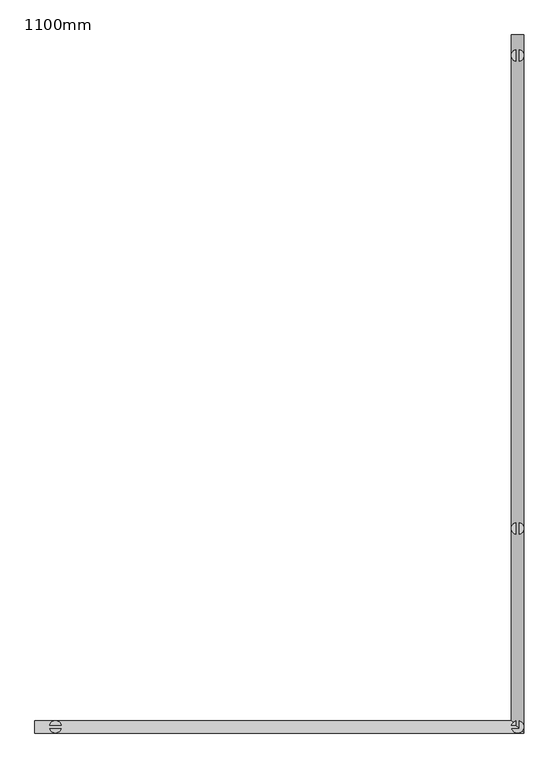
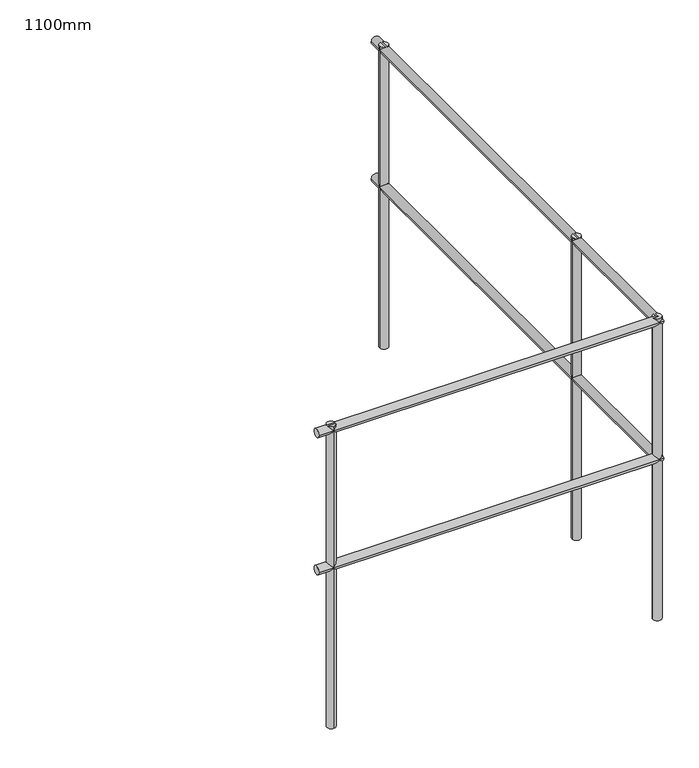
"""IFC4 building model written with IfcOpenShell, lengths in millimetres: railing geometry, 1100mm."""

from ifc_helpers import new_model, si_unit, point, frame, frame_2d, origin, place, context, project, spatial, circle_curve, ellipse_curve, trimmed, segment, composite_curve, outline, extrude, source, transform, mapped, element, save
from ifc_brep_helpers import plane_surface, cylinder_surface, advanced_brep


def railing_1100mm_da86e9fc(model_context):
    return source(origin(), model_context, "Body", "SolidModel", [
        advanced_brep(
        [(11414.7052251, 14979.5208589, 4745.0), (11384.7052251, 14979.5208589, 4745.0), (10225.0, 13282.0208589, 4745.0), (10225.0, 13312.0208589, 4745.0), (11414.7052251, 13282.0208589, 4745.0), (11384.7052251, 13312.0208589, 4745.0)],
        [
            (0, 1, circle_curve(frame((11399.7052251, 14979.5208589, 4745.0), z_axis=(0.0, 1.0, 0.0), x_axis=(-1.0, 0.0, 0.0)), 15.0)),
            (1, 0, circle_curve(frame((11399.7052251, 14979.5208589, 4745.0), z_axis=(0.0, 1.0, 0.0), x_axis=(-1.0, 0.0, 0.0)), 15.0)),
            (2, 3, circle_curve(frame((10225.0, 13297.0208589, 4745.0), z_axis=(-1.0, 0.0, 0.0), x_axis=(0.0, 1.0, 0.0)), 15.0)),
            (3, 2, circle_curve(frame((10225.0, 13297.0208589, 4745.0), z_axis=(-1.0, 0.0, 0.0), x_axis=(0.0, 1.0, 0.0)), 15.0)),
            (0, 4),
            (4, 5, ellipse_curve(frame((11399.7052251, 13297.0208589, 4745.0), z_axis=(0.7071067811865493, 0.7071067811865457, 0.0), x_axis=(-0.7071067811865457, 0.7071067811865493, 0.0)), 21.2132034, 15.0)),
            (5, 1),
            (5, 4, ellipse_curve(frame((11399.7052251, 13297.0208589, 4745.0), z_axis=(0.7071067811865493, 0.7071067811865457, 0.0), x_axis=(-0.7071067811865457, 0.7071067811865493, 0.0)), 21.2132034, 15.0)),
            (4, 2),
            (3, 5),
        ],
        [
            plane_surface(frame((11399.7052251, 14979.5208589, 4760.0), z_axis=(0.0, 1.0, 0.0), x_axis=(0.0, 0.0, -1.0))),
            plane_surface(frame((10225.0, 13297.0208589, 4760.0), z_axis=(-1.0, 0.0, 0.0), x_axis=(0.0, -1.0, 0.0))),
            cylinder_surface(frame((11399.7052251, 14979.5208589, 4745.0), z_axis=(0.0, 1.0, 0.0), x_axis=(-1.0, 0.0, 0.0)), 15.0),
            cylinder_surface(frame((11399.7052251, 13297.0208589, 4745.0), z_axis=(1.0, 0.0, 0.0), x_axis=(0.0, 1.0, 0.0)), 15.0),
        ],
        [
            (0, [[1, 2]]),
            (1, [[3, 4]]),
            (2, [[-1, 5, 6, 7]]),
            (2, [[-2, -7, 8, -5]]),
            (3, [[-6, 9, -4, 10]]),
            (3, [[-8, -10, -3, -9]]),
        ],
    ),
        advanced_brep(
        [(11414.7052251, 14979.5208589, 5245.0), (11384.7052251, 14979.5208589, 5245.0), (11414.7052251, 13282.0208589, 5245.0), (11384.7052251, 13312.0208589, 5245.0), (10225.0, 13282.0208589, 5245.0), (10225.0, 13312.0208589, 5245.0)],
        [
            (0, 1, circle_curve(frame((11399.7052251, 14979.5208589, 5245.0), z_axis=(0.0, 1.0, 0.0), x_axis=(-1.0, 0.0, 0.0)), 15.0)),
            (1, 0, circle_curve(frame((11399.7052251, 14979.5208589, 5245.0), z_axis=(0.0, 1.0, 0.0), x_axis=(-1.0, 0.0, 0.0)), 15.0)),
            (0, 2),
            (2, 3, ellipse_curve(frame((11399.7052251, 13297.0208589, 5245.0), z_axis=(0.7071067811865493, 0.7071067811865457, 0.0), x_axis=(-0.7071067811865457, 0.7071067811865493, 0.0)), 21.2132034, 15.0)),
            (3, 1),
            (3, 2, ellipse_curve(frame((11399.7052251, 13297.0208589, 5245.0), z_axis=(0.7071067811865493, 0.7071067811865457, 0.0), x_axis=(-0.7071067811865457, 0.7071067811865493, 0.0)), 21.2132034, 15.0)),
            (4, 5, circle_curve(frame((10225.0, 13297.0208589, 5245.0), z_axis=(-1.0, 0.0, 0.0), x_axis=(0.0, 1.0, 0.0)), 15.0)),
            (5, 4, circle_curve(frame((10225.0, 13297.0208589, 5245.0), z_axis=(-1.0, 0.0, 0.0), x_axis=(0.0, 1.0, 0.0)), 15.0)),
            (2, 4),
            (5, 3),
        ],
        [
            plane_surface(frame((11399.7052251, 14979.5208589, 5260.0), z_axis=(0.0, 1.0, 0.0), x_axis=(0.0, 0.0, -1.0))),
            cylinder_surface(frame((11399.7052251, 14979.5208589, 5245.0), z_axis=(0.0, 1.0, 0.0), x_axis=(-1.0, 0.0, 0.0)), 15.0),
            plane_surface(frame((10225.0, 13297.0208589, 5260.0), z_axis=(-1.0, 0.0, 0.0), x_axis=(0.0, -1.0, 0.0))),
            cylinder_surface(frame((11399.7052251, 13297.0208589, 5245.0), z_axis=(1.0, 0.0, 0.0), x_axis=(0.0, 1.0, 0.0)), 15.0),
        ],
        [
            (0, [[1, 2]]),
            (1, [[-1, 3, 4, 5]]),
            (1, [[-2, -5, 6, -3]]),
            (2, [[7, 8]]),
            (3, [[-4, 9, -8, 10]]),
            (3, [[-6, -10, -7, -9]]),
        ],
    ),
        extrude(outline(composite_curve([segment(trimmed(circle_curve(frame_2d((11399.7052251, 13779.5208589)), 15.0), [point((11384.7052251, 13779.5208589))], [point((11414.7052251, 13779.5208589))], False, "CARTESIAN"), True, "CONTINUOUS"), segment(trimmed(circle_curve(frame_2d((11399.7052251, 13779.5208589)), 15.0), [point((11414.7052251, 13779.5208589))], [point((11384.7052251, 13779.5208589))], False, "CARTESIAN"), True, "CONTINUOUS")], self_intersect=False)), frame((0.0, 0.0, 4160.0), z_axis=(0.0, 0.0, 1.0), x_axis=(1.0, 0.0, 0.0)), (0.0, 0.0, 1.0), 1100.0),
        extrude(outline(composite_curve([segment(trimmed(circle_curve(frame_2d((11399.7052251, 13297.0208589)), 15.0), [point((11384.7052251, 13297.0208589))], [point((11414.7052251, 13297.0208589))], False, "CARTESIAN"), True, "CONTINUOUS"), segment(trimmed(circle_curve(frame_2d((11399.7052251, 13297.0208589)), 15.0), [point((11414.7052251, 13297.0208589))], [point((11384.7052251, 13297.0208589))], False, "CARTESIAN"), True, "CONTINUOUS")], self_intersect=False)), frame((0.0, 0.0, 4160.0), z_axis=(0.0, 0.0, 1.0), x_axis=(1.0, 0.0, 0.0)), (0.0, 0.0, 1.0), 1100.0),
        extrude(outline(composite_curve([segment(trimmed(circle_curve(frame_2d((10275.0, 13297.0208589)), 15.0), [point((10275.0, 13312.0208589))], [point((10275.0, 13282.0208589))], False, "CARTESIAN"), True, "CONTINUOUS"), segment(trimmed(circle_curve(frame_2d((10275.0, 13297.0208589)), 15.0), [point((10275.0, 13282.0208589))], [point((10275.0, 13312.0208589))], False, "CARTESIAN"), True, "CONTINUOUS")], self_intersect=False)), frame((0.0, 0.0, 4160.0), z_axis=(0.0, 0.0, 1.0), x_axis=(1.0, 0.0, 0.0)), (0.0, 0.0, 1.0), 1100.0),
        extrude(outline(composite_curve([segment(trimmed(circle_curve(frame_2d((11399.7052251, 14929.5208589)), 15.0), [point((11384.7052251, 14929.5208589))], [point((11414.7052251, 14929.5208589))], False, "CARTESIAN"), True, "CONTINUOUS"), segment(trimmed(circle_curve(frame_2d((11399.7052251, 14929.5208589)), 15.0), [point((11414.7052251, 14929.5208589))], [point((11384.7052251, 14929.5208589))], False, "CARTESIAN"), True, "CONTINUOUS")], self_intersect=False)), frame((0.0, 0.0, 4160.0), z_axis=(0.0, 0.0, 1.0), x_axis=(1.0, 0.0, 0.0)), (0.0, 0.0, 1.0), 1100.0),
    ])


if __name__ == "__main__":
    model = new_model("IFC4")
    model_context = context("Model", 3, world=origin())
    ifc_project = project(units=[si_unit("LENGTHUNIT", "METRE", prefix="MILLI")], contexts=[model_context])
    site = spatial("IfcSite", under=ifc_project)
    building = spatial("IfcBuilding", under=site)
    placement = place(None, origin())
    railing_1100mm_shape = railing_1100mm_da86e9fc(model_context)
    element("IfcRailing", 1, ObjectType="1100mm", at=placement, inside=building, context=model_context, shape_type="MappedRepresentation", body=[
        mapped(railing_1100mm_shape, transform((0.0, 0.0, 0.0), x_axis=(1.0, 0.0, 0.0), y_axis=(0.0, 1.0, 0.0), z_axis=(0.0, 0.0, 1.0))),
    ])
    save(model, "model.ifc")
